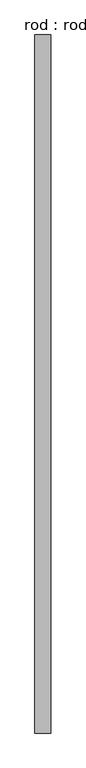
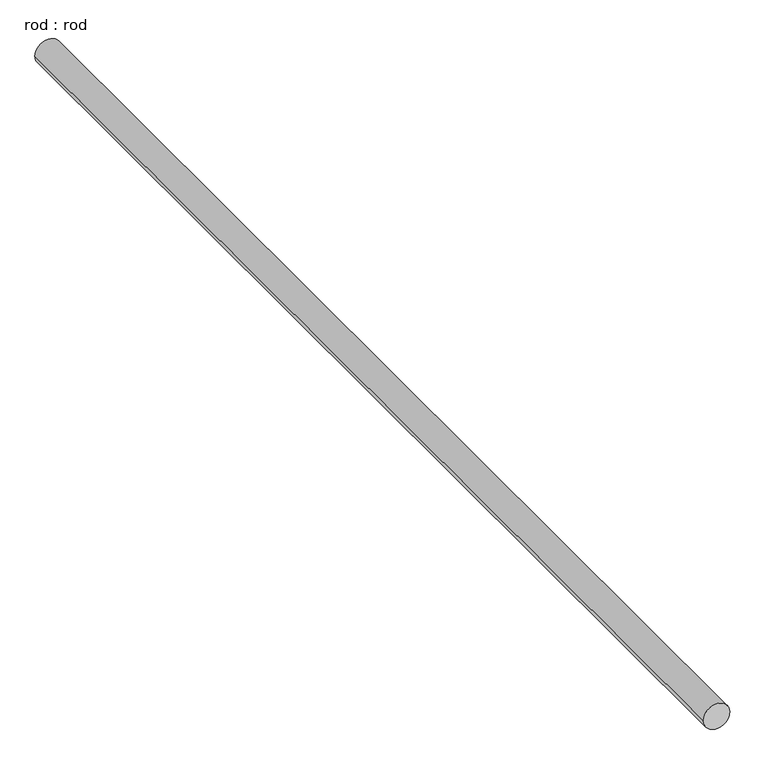
"""IFC4 building model written with IfcOpenShell, lengths in millimetres: proxy geometry, rod : rod."""

from ifc_helpers import new_model, si_unit, point, frame, frame_2d, origin, place, context, project, spatial, circle_curve, trimmed, segment, composite_curve, outline, extrude, source, transform, mapped, element, save


def rod_rod_02b657ae(model_context):
    return source(origin(), model_context, "Body", "SweptSolid", [
        extrude(outline(composite_curve([segment(trimmed(circle_curve(frame_2d((0.0108462, 0.0)), 200.0), [point((0.0108462, 200.0))], [point((0.0108462, -200.0))], False, "CARTESIAN"), True, "CONTINUOUS"), segment(trimmed(circle_curve(frame_2d((0.0108462, 0.0)), 200.0), [point((0.0108462, -200.0))], [point((0.0108462, 200.0))], False, "CARTESIAN"), True, "CONTINUOUS")], self_intersect=False)), frame((0.0, -4682.3675584, 0.0), z_axis=(0.0, 1.0, 0.0), x_axis=(0.0, 0.0, 1.0)), (0.0, 0.0, 1.0), 17550.1923475),
    ])


if __name__ == "__main__":
    model = new_model("IFC4")
    model_context = context("Model", 3, world=origin())
    ifc_project = project(units=[si_unit("LENGTHUNIT", "METRE", prefix="MILLI")], contexts=[model_context])
    site = spatial("IfcSite", under=ifc_project)
    building = spatial("IfcBuilding", under=site)
    placement = place(None, origin())
    rod_rod_shape = rod_rod_02b657ae(model_context)
    element("IfcBuildingElementProxy", 1, Name="rod : rod", ObjectType="rod : rod", at=placement, inside=building, context=model_context, shape_type="MappedRepresentation", body=[
        mapped(rod_rod_shape, transform((0.0, 0.0, 0.0), x_axis=(1.0, 0.0, 0.0), y_axis=(0.0, 1.0, 0.0), z_axis=(0.0, 0.0, 1.0))),
    ])
    save(model, "model.ifc")

# Revit data of these elements
# Type "rod : rod"
#   Default Elevation = 0
